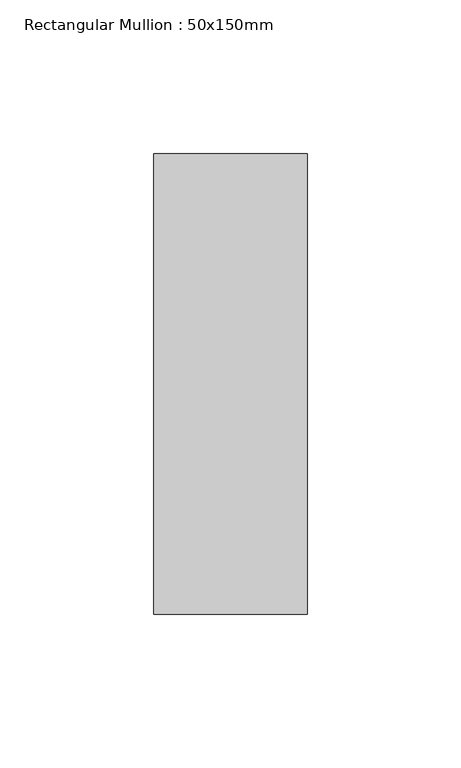
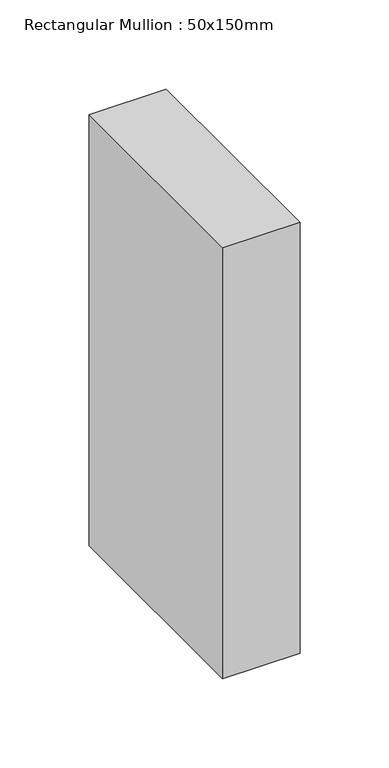
"""IFC4 building model written with IfcOpenShell, lengths in millimetres: member geometry, Rectangular Mullion : 50x150mm."""

from ifc_helpers import new_model, si_unit, frame, origin, place, context, project, spatial, polyline, outline, extrude, source, transform, mapped, element, save


def rectangular_mullion_50x150mm_3d88505a(model_context):
    return source(origin(), model_context, "Body", "SweptSolid", [
        extrude(outline(polyline([(0.0, 75.0), (0.0, -75.0), (-50.0, -75.0), (-50.0, 75.0), (0.0, 75.0)])), frame((0.0, 0.0, -294.9999997), z_axis=(0.0, 0.0, 1.0), x_axis=(1.0, 0.0, 0.0)), (0.0, 0.0, 1.0), 294.9999997),
    ])


if __name__ == "__main__":
    model = new_model("IFC4")
    model_context = context("Model", 3, world=origin())
    ifc_project = project(units=[si_unit("LENGTHUNIT", "METRE", prefix="MILLI")], contexts=[model_context])
    site = spatial("IfcSite", under=ifc_project)
    building = spatial("IfcBuilding", under=site)
    placement = place(None, origin())
    rectangular_mullion_50x150mm_shape = rectangular_mullion_50x150mm_3d88505a(model_context)
    element("IfcMember", 1, ObjectType="Rectangular Mullion : 50x150mm", at=placement, inside=building, context=model_context, shape_type="MappedRepresentation", body=[
        mapped(rectangular_mullion_50x150mm_shape, transform((0.0, 0.0, 0.0), x_axis=(1.0, 0.0, 0.0), y_axis=(0.0, 1.0, 0.0), z_axis=(0.0, 0.0, 1.0))),
    ])
    save(model, "model.ifc")

# Revit data of these elements
# Type "Rectangular Mullion : 50x150mm"
#   Keynote = "H11"
#   built-in parameter 1007304 = 0.492126 (stored number, unit not read)
#   built-in parameter 1007301 = 0.082021 (stored number, unit not read)
#   built-in parameter 1007300 = 0.082021 (stored number, unit not read)
# Element 1 (IfcMember, "Rectangular Mullion : 50x150mm")
#   Materials on its faces: "Aluminium"
# Materials
#   "Aluminium": class "Metal", colour RGB 247 247 247, transparency 0, Description = "Aluminium 6061", Cost = 0
